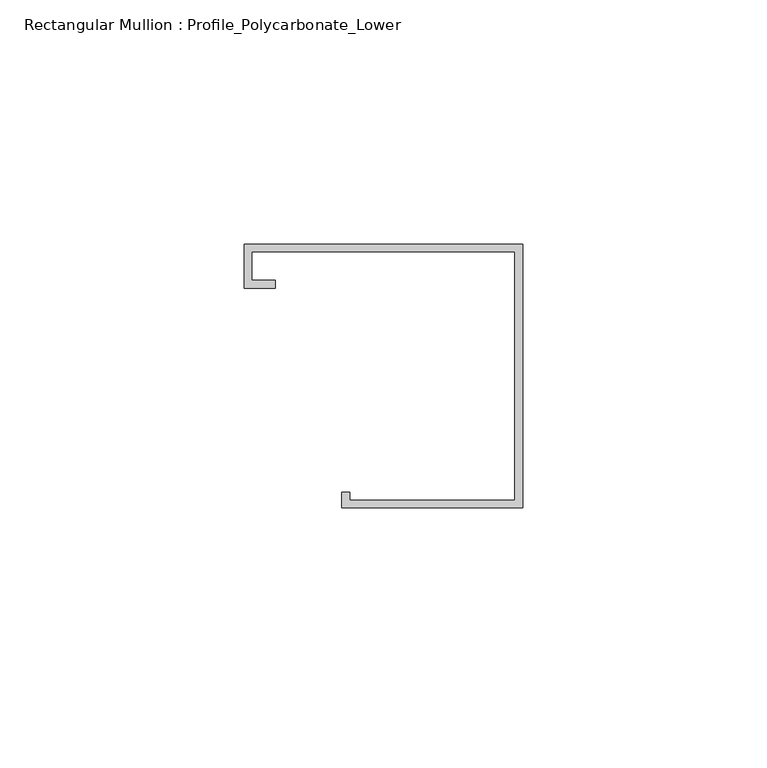
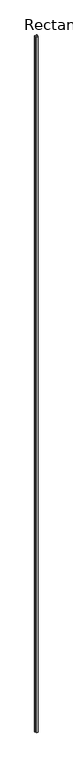
"""IFC4 building model written with IfcOpenShell, lengths in millimetres: member geometry, Rectangular Mullion : Profile_Polycarbonate_Lower."""

from ifc_helpers import new_model, si_unit, frame, origin, place, context, project, spatial, polyline, outline, extrude, source, transform, mapped, element, save


def rectangular_mullion_profile_polycarbonate_lower_d4813d95(model_context):
    return source(origin(), model_context, "Body", "SweptSolid", [
        extrude(outline(polyline([(0.0, 28.984575), (0.0, -25.015825), (-36.9824, -25.015825), (-36.9824, -21.840825), (-35.3949, -21.840825), (-35.3949, -23.428325), (-1.5875, -23.428325), (-1.5875, 27.397075), (-55.4101, 27.397075), (-55.4101, 21.580475), (-50.6476, 21.580475), (-50.6476, 19.992975), (-56.9976, 19.992975), (-56.9976, 28.984575), (0.0, 28.984575)])), frame((0.0, 0.0, -18548.5024), z_axis=(0.0, 0.0, 1.0), x_axis=(1.0, 0.0, 0.0)), (0.0, 0.0, 1.0), 18548.5024),
    ])


if __name__ == "__main__":
    model = new_model("IFC4")
    model_context = context("Model", 3, world=origin())
    ifc_project = project(units=[si_unit("LENGTHUNIT", "METRE", prefix="MILLI")], contexts=[model_context])
    site = spatial("IfcSite", under=ifc_project)
    building = spatial("IfcBuilding", under=site)
    placement = place(None, origin())
    rectangular_mullion_profile_polycarbonate_lower_shape = rectangular_mullion_profile_polycarbonate_lower_d4813d95(model_context)
    element("IfcMember", 1, ObjectType="Rectangular Mullion : Profile_Polycarbonate_Lower", at=placement, inside=building, context=model_context, shape_type="MappedRepresentation", body=[
        mapped(rectangular_mullion_profile_polycarbonate_lower_shape, transform((0.0, 0.0, 0.0), x_axis=(1.0, 0.0, 0.0), y_axis=(0.0, 1.0, 0.0), z_axis=(0.0, 0.0, 1.0))),
    ])
    save(model, "model.ifc")

# Revit data of these elements
# Type "Rectangular Mullion : Profile_Polycarbonate_Lower"
#   built-in parameter 1007322 = 0.177167 (stored number, unit not read)
#   built-in parameter 1007321 = 0 (stored number, unit not read)
#   built-in parameter 1007320 = 0.00520833 (stored number, unit not read)
